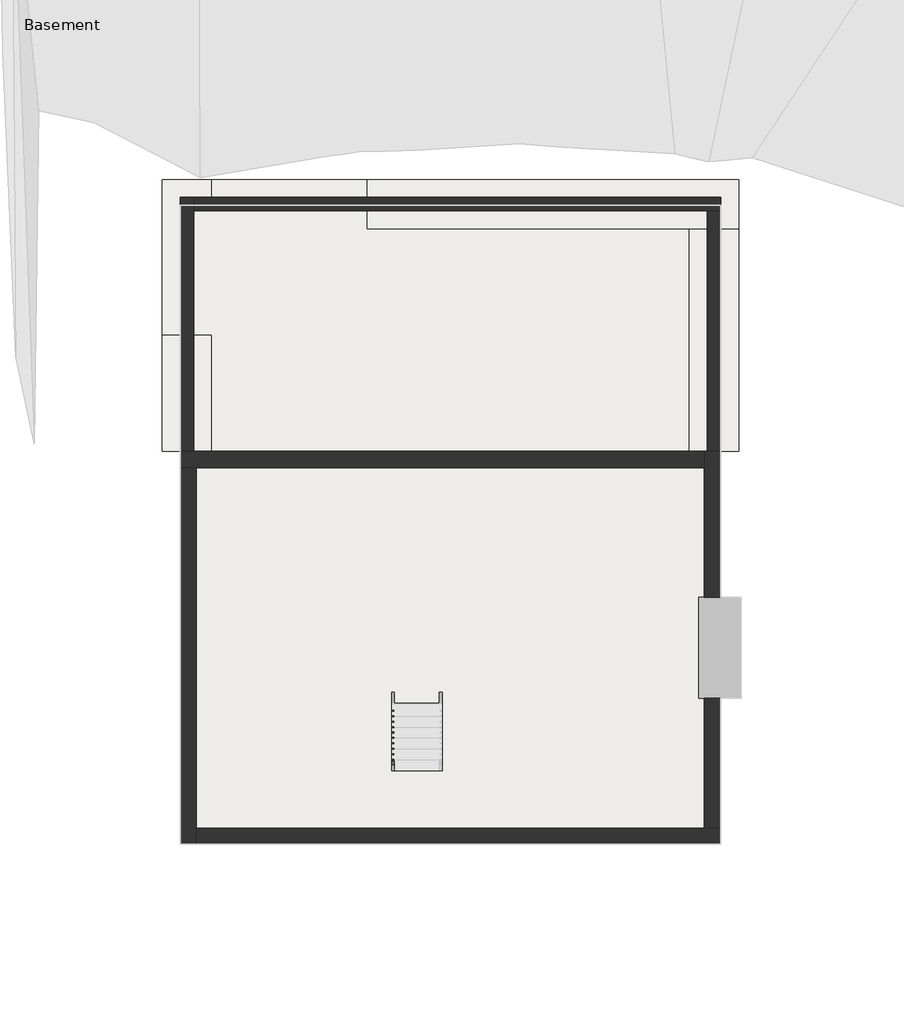
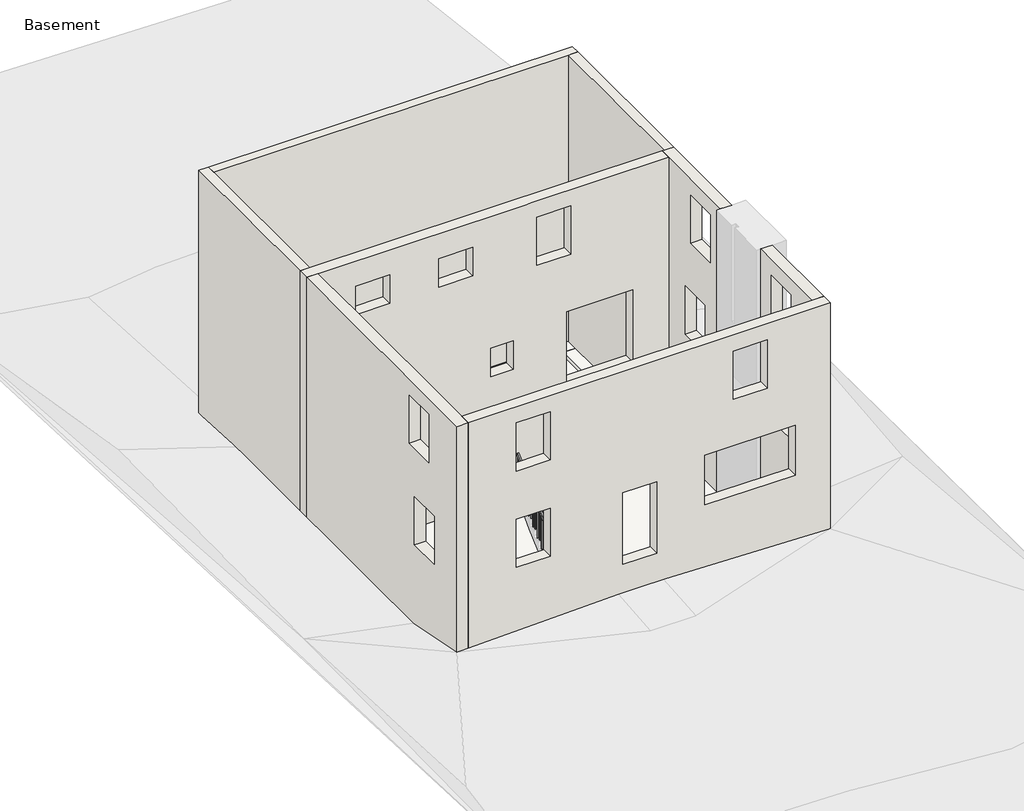
# One storey, part 1 of 2: 8 walls, 3 footings, 2 slabs, 1 railing.
"""IFC4 building model written with IfcOpenShell, lengths in millimetres."""

from ifc_helpers import new_model, si_unit, frame, origin, place, context, project, spatial, polyline, outline, extrude, faceted_brep, element, save

model = new_model("IFC4")

# Units and contexts
model_context = context("Model", 3, world=origin())
ifc_project = project(units=[si_unit("LENGTHUNIT", "METRE", prefix="MILLI")], contexts=[model_context])

# Site, building, storey
site = spatial("IfcSite", under=ifc_project)
building = spatial("IfcBuilding", under=site)
storey = spatial("IfcBuildingStorey", under=building, Name="Basement", Elevation=-2667.0)

# Footings
placement = place(None, origin())
element("IfcFooting", 1, ObjectType="Bearing Footing - 36\" x 12\"", at=placement, inside=storey, context=model_context, shape_type="Brep", body=[
    faceted_brep([(-5404.9803068, 3152.0888758, -2667.0), (-6319.3803068, 3152.0888758, -2667.0), (-6319.3803068, 3152.0888758, -2971.8), (-5404.9803068, 3152.0888758, -2971.8), (-6319.3803068, 5311.0888758, -2667.0), (-5404.9803068, 5311.0888758, -2667.0), (-5404.9803068, 5311.0888758, -2971.8), (-6319.3803068, 5311.0888758, -2971.8)], [[[0, 1, 2, 3]], [[4, 5, 6, 7]], [[0, 5, 4, 1]], [[2, 1, 4, 7]], [[3, 2, 7, 6]], [[0, 3, 6, 5]]]),
    faceted_brep([(-5404.9803068, 5311.0888758, -3124.2), (-6319.3803068, 5311.0888758, -3124.2), (-6319.3803068, 5311.0888758, -3429.0), (-5404.9803068, 5311.0888758, -3429.0), (-5404.9803068, 7292.2888758, -3124.2), (-5404.9803068, 8206.6888758, -3124.2), (-6319.3803068, 8206.6888758, -3124.2), (-6319.3803068, 8206.6888758, -3429.0), (-5404.9803068, 8206.6888758, -3429.0), (-5404.9803068, 7292.2888758, -3429.0)], [[[0, 1, 2, 3]], [[0, 4, 5, 6, 1]], [[2, 1, 6, 7]], [[3, 2, 7, 8, 9]], [[0, 3, 9, 8, 5, 4]], [[6, 5, 8, 7]]]),
])
element("IfcFooting", 2, ObjectType="Bearing Footing - 36\" x 12\"", at=placement, inside=storey, context=model_context, shape_type="Brep", body=[
    faceted_brep([(-2509.3803068, 8206.6888758, -3429.0), (-2509.3803068, 8206.6888758, -3124.2), (-2509.3803068, 7292.2888758, -3124.2), (-2509.3803068, 7292.2888758, -3429.0), (-5404.9803068, 8206.6888758, -3124.2), (-5404.9803068, 7292.2888758, -3124.2), (-5404.9803068, 8206.6888758, -3429.0), (-5404.9803068, 7292.2888758, -3429.0)], [[[0, 1, 2, 3]], [[2, 1, 4, 5]], [[1, 0, 6, 4]], [[0, 3, 7, 6]], [[3, 2, 5, 7]], [[5, 4, 6, 7]]]),
    faceted_brep([(-2509.3803068, 8206.6888758, -2667.0), (-2509.3803068, 8206.6888758, -2971.8), (-2509.3803068, 7292.2888758, -2971.8), (-2509.3803068, 7292.2888758, -2667.0), (4399.4196932, 8206.6888758, -2667.0), (3485.0196932, 7292.2888758, -2667.0), (4399.4196932, 7292.2888758, -2667.0), (4399.4196932, 8206.6888758, -2971.8), (4399.4196932, 7292.2888758, -2971.8), (3485.0196932, 7292.2888758, -2971.8)], [[[0, 1, 2, 3]], [[4, 0, 3, 5, 6]], [[1, 0, 4, 7]], [[2, 1, 7, 8, 9]], [[3, 2, 9, 8, 6, 5]], [[4, 6, 8, 7]]]),
])
element("IfcFooting", 3, ObjectType="Bearing Footing - 36\" x 12\"", at=placement, inside=storey, context=model_context, shape_type="SweptSolid", body=[
    extrude(outline(polyline([(4399.4196932, 3152.0888758), (3485.0196932, 3152.0888758), (3485.0196932, 7292.2888758), (4399.4196932, 7292.2888758), (4399.4196932, 3152.0888758)])), frame((0.0, 0.0, -2971.8), z_axis=(0.0, 0.0, 1.0), x_axis=(1.0, 0.0, 0.0)), (0.0, 0.0, 1.0), 304.8),
])

# Railing
element("IfcRailing", 4, ObjectType="Handrail - Rectangular", at=placement, inside=storey, context=model_context, shape_type="SweptSolid", body=[
    extrude(outline(polyline([(-2791.5111242, -1631.7331862), (-2791.5111242, -1562.1), (-149.9111242, 914.4), (-149.9111242, 844.7668138), (-2791.5111242, -1631.7331862)])), frame((-2052.1803068, 0.0, 0.0), z_axis=(1.0, 0.0, 0.0), x_axis=(0.0, 1.0, 0.0)), (0.0, 0.0, 1.0), 50.8),
    extrude(outline(polyline([(-241.9861242, 758.4465013), (-241.9861242, -190.5), (-261.0361242, -190.5), (-261.0361242, 740.5871263), (-241.9861242, 758.4465013)])), frame((-2036.3053068, 0.0, 0.0), z_axis=(1.0, 0.0, 0.0), x_axis=(0.0, 1.0, 0.0)), (0.0, 0.0, 1.0), 19.05),
    extrude(outline(polyline([(-343.5861242, 663.1965013), (-343.5861242, -190.5), (-362.6361242, -190.5), (-362.6361242, 645.3371263), (-343.5861242, 663.1965013)])), frame((-2036.3053068, 0.0, 0.0), z_axis=(1.0, 0.0, 0.0), x_axis=(0.0, 1.0, 0.0)), (0.0, 0.0, 1.0), 19.05),
    extrude(outline(polyline([(-445.1861242, 567.9465013), (-445.1861242, -381.0), (-464.2361242, -381.0), (-464.2361242, 550.0871263), (-445.1861242, 567.9465013)])), frame((-2036.3053068, 0.0, 0.0), z_axis=(1.0, 0.0, 0.0), x_axis=(0.0, 1.0, 0.0)), (0.0, 0.0, 1.0), 19.05),
    extrude(outline(polyline([(-546.7861242, 472.6965013), (-546.7861242, -381.0), (-565.8361242, -381.0), (-565.8361242, 454.8371263), (-546.7861242, 472.6965013)])), frame((-2036.3053068, 0.0, 0.0), z_axis=(1.0, 0.0, 0.0), x_axis=(0.0, 1.0, 0.0)), (0.0, 0.0, 1.0), 19.05),
    extrude(outline(polyline([(-648.3861242, 377.4465013), (-648.3861242, -571.5), (-667.4361242, -571.5), (-667.4361242, 359.5871263), (-648.3861242, 377.4465013)])), frame((-2036.3053068, 0.0, 0.0), z_axis=(1.0, 0.0, 0.0), x_axis=(0.0, 1.0, 0.0)), (0.0, 0.0, 1.0), 19.05),
    extrude(outline(polyline([(-749.9861242, 282.1965013), (-749.9861242, -571.5), (-769.0361242, -571.5), (-769.0361242, 264.3371263), (-749.9861242, 282.1965013)])), frame((-2036.3053068, 0.0, 0.0), z_axis=(1.0, 0.0, 0.0), x_axis=(0.0, 1.0, 0.0)), (0.0, 0.0, 1.0), 19.05),
    extrude(outline(polyline([(-851.5861242, 186.9465013), (-851.5861242, -762.0), (-870.6361242, -762.0), (-870.6361242, 169.0871263), (-851.5861242, 186.9465013)])), frame((-2036.3053068, 0.0, 0.0), z_axis=(1.0, 0.0, 0.0), x_axis=(0.0, 1.0, 0.0)), (0.0, 0.0, 1.0), 19.05),
    extrude(outline(polyline([(-953.1861242, 91.6965013), (-953.1861242, -762.0), (-972.2361242, -762.0), (-972.2361242, 73.8371263), (-953.1861242, 91.6965013)])), frame((-2036.3053068, 0.0, 0.0), z_axis=(1.0, 0.0, 0.0), x_axis=(0.0, 1.0, 0.0)), (0.0, 0.0, 1.0), 19.05),
    extrude(outline(polyline([(-1054.7861242, -3.5534987), (-1054.7861242, -952.5), (-1073.8361242, -952.5), (-1073.8361242, -21.4128737), (-1054.7861242, -3.5534987)])), frame((-2036.3053068, 0.0, 0.0), z_axis=(1.0, 0.0, 0.0), x_axis=(0.0, 1.0, 0.0)), (0.0, 0.0, 1.0), 19.05),
    extrude(outline(polyline([(-1156.3861242, -98.8034987), (-1156.3861242, -952.5), (-1175.4361242, -952.5), (-1175.4361242, -116.6628737), (-1156.3861242, -98.8034987)])), frame((-2036.3053068, 0.0, 0.0), z_axis=(1.0, 0.0, 0.0), x_axis=(0.0, 1.0, 0.0)), (0.0, 0.0, 1.0), 19.05),
    extrude(outline(polyline([(-1257.9861242, -194.0534987), (-1257.9861242, -1143.0), (-1277.0361242, -1143.0), (-1277.0361242, -211.9128737), (-1257.9861242, -194.0534987)])), frame((-2036.3053068, 0.0, 0.0), z_axis=(1.0, 0.0, 0.0), x_axis=(0.0, 1.0, 0.0)), (0.0, 0.0, 1.0), 19.05),
    extrude(outline(polyline([(-1359.5861242, -289.3034987), (-1359.5861242, -1143.0), (-1378.6361242, -1143.0), (-1378.6361242, -307.1628737), (-1359.5861242, -289.3034987)])), frame((-2036.3053068, 0.0, 0.0), z_axis=(1.0, 0.0, 0.0), x_axis=(0.0, 1.0, 0.0)), (0.0, 0.0, 1.0), 19.05),
    extrude(outline(polyline([(-1461.1861242, -384.5534987), (-1461.1861242, -1333.5), (-1480.2361242, -1333.5), (-1480.2361242, -402.4128737), (-1461.1861242, -384.5534987)])), frame((-2036.3053068, 0.0, 0.0), z_axis=(1.0, 0.0, 0.0), x_axis=(0.0, 1.0, 0.0)), (0.0, 0.0, 1.0), 19.05),
    extrude(outline(polyline([(-1562.7861242, -479.8034987), (-1562.7861242, -1333.5), (-1581.8361242, -1333.5), (-1581.8361242, -497.6628737), (-1562.7861242, -479.8034987)])), frame((-2036.3053068, 0.0, 0.0), z_axis=(1.0, 0.0, 0.0), x_axis=(0.0, 1.0, 0.0)), (0.0, 0.0, 1.0), 19.05),
    extrude(outline(polyline([(-1664.3861242, -575.0534987), (-1664.3861242, -1524.0), (-1683.4361242, -1524.0), (-1683.4361242, -592.9128737), (-1664.3861242, -575.0534987)])), frame((-2036.3053068, 0.0, 0.0), z_axis=(1.0, 0.0, 0.0), x_axis=(0.0, 1.0, 0.0)), (0.0, 0.0, 1.0), 19.05),
    extrude(outline(polyline([(-1765.9861242, -670.3034987), (-1765.9861242, -1524.0), (-1785.0361242, -1524.0), (-1785.0361242, -688.1628737), (-1765.9861242, -670.3034987)])), frame((-2036.3053068, 0.0, 0.0), z_axis=(1.0, 0.0, 0.0), x_axis=(0.0, 1.0, 0.0)), (0.0, 0.0, 1.0), 19.05),
    extrude(outline(polyline([(-1867.5861242, -765.5534987), (-1867.5861242, -1714.5), (-1886.6361242, -1714.5), (-1886.6361242, -783.4128737), (-1867.5861242, -765.5534987)])), frame((-2036.3053068, 0.0, 0.0), z_axis=(1.0, 0.0, 0.0), x_axis=(0.0, 1.0, 0.0)), (0.0, 0.0, 1.0), 19.05),
    extrude(outline(polyline([(-1969.1861242, -860.8034987), (-1969.1861242, -1714.5), (-1988.2361242, -1714.5), (-1988.2361242, -878.6628737), (-1969.1861242, -860.8034987)])), frame((-2036.3053068, 0.0, 0.0), z_axis=(1.0, 0.0, 0.0), x_axis=(0.0, 1.0, 0.0)), (0.0, 0.0, 1.0), 19.05),
    extrude(outline(polyline([(-2070.7861242, -956.0534987), (-2070.7861242, -1905.0), (-2089.8361242, -1905.0), (-2089.8361242, -973.9128737), (-2070.7861242, -956.0534987)])), frame((-2036.3053068, 0.0, 0.0), z_axis=(1.0, 0.0, 0.0), x_axis=(0.0, 1.0, 0.0)), (0.0, 0.0, 1.0), 19.05),
    extrude(outline(polyline([(-2172.3861242, -1051.3034987), (-2172.3861242, -1905.0), (-2191.4361242, -1905.0), (-2191.4361242, -1069.1628737), (-2172.3861242, -1051.3034987)])), frame((-2036.3053068, 0.0, 0.0), z_axis=(1.0, 0.0, 0.0), x_axis=(0.0, 1.0, 0.0)), (0.0, 0.0, 1.0), 19.05),
    extrude(outline(polyline([(-2273.9861242, -1146.5534987), (-2273.9861242, -2095.5), (-2293.0361242, -2095.5), (-2293.0361242, -1164.4128737), (-2273.9861242, -1146.5534987)])), frame((-2036.3053068, 0.0, 0.0), z_axis=(1.0, 0.0, 0.0), x_axis=(0.0, 1.0, 0.0)), (0.0, 0.0, 1.0), 19.05),
    extrude(outline(polyline([(-2375.5861242, -1241.8034987), (-2375.5861242, -2095.5), (-2394.6361242, -2095.5), (-2394.6361242, -1259.6628737), (-2375.5861242, -1241.8034987)])), frame((-2036.3053068, 0.0, 0.0), z_axis=(1.0, 0.0, 0.0), x_axis=(0.0, 1.0, 0.0)), (0.0, 0.0, 1.0), 19.05),
    extrude(outline(polyline([(-2477.1861242, -1337.0534987), (-2477.1861242, -2286.0), (-2496.2361242, -2286.0), (-2496.2361242, -1354.9128737), (-2477.1861242, -1337.0534987)])), frame((-2036.3053068, 0.0, 0.0), z_axis=(1.0, 0.0, 0.0), x_axis=(0.0, 1.0, 0.0)), (0.0, 0.0, 1.0), 19.05),
    extrude(outline(polyline([(-2578.7861242, -1432.3034987), (-2578.7861242, -2286.0), (-2597.8361242, -2286.0), (-2597.8361242, -1450.1628737), (-2578.7861242, -1432.3034987)])), frame((-2036.3053068, 0.0, 0.0), z_axis=(1.0, 0.0, 0.0), x_axis=(0.0, 1.0, 0.0)), (0.0, 0.0, 1.0), 19.05),
    extrude(outline(polyline([(-2680.3861242, -1527.5534987), (-2680.3861242, -2476.5), (-2699.4361242, -2476.5), (-2699.4361242, -1545.4128737), (-2680.3861242, -1527.5534987)])), frame((-2036.3053068, 0.0, 0.0), z_axis=(1.0, 0.0, 0.0), x_axis=(0.0, 1.0, 0.0)), (0.0, 0.0, 1.0), 19.05),
    extrude(outline(polyline([(-149.9111242, 844.7668138), (-149.9111242, -190.5), (-168.9611242, -190.5), (-168.9611242, 826.9074388), (-149.9111242, 844.7668138)])), frame((-2036.3053068, 0.0, 0.0), z_axis=(1.0, 0.0, 0.0), x_axis=(0.0, 1.0, 0.0)), (0.0, 0.0, 1.0), 19.05),
    extrude(outline(polyline([(-2772.4611242, -1613.8738112), (-2772.4611242, -2476.5), (-2791.5111242, -2476.5), (-2791.5111242, -1631.7331862), (-2772.4611242, -1613.8738112)])), frame((-2036.3053068, 0.0, 0.0), z_axis=(1.0, 0.0, 0.0), x_axis=(0.0, 1.0, 0.0)), (0.0, 0.0, 1.0), 19.05),
])

# Slabs
element("IfcSlab", 5, ObjectType="Pad 1", at=placement, inside=storey, context=model_context, shape_type="SweptSolid", body=[
    extrude(outline(polyline([(4069.2196932, 434.2888758), (4450.2196932, 434.2888758), (4450.2196932, -1445.3111242), (4069.2196932, -1445.3111242), (4069.2196932, -4163.1111242), (-5989.1803068, -4163.1111242), (-5989.1803068, 3152.0888758), (4069.2196932, 3152.0888758), (4069.2196932, 434.2888758)])), frame((0.0, 0.0, -3073.4), z_axis=(0.0, 0.0, 1.0), x_axis=(1.0, 0.0, 0.0)), (0.0, 0.0, 1.0), 304.8),
])
element("IfcSlab", 6, ObjectType="Pad 1", at=placement, inside=storey, context=model_context, shape_type="SweptSolid", body=[
    extrude(outline(polyline([(-5989.1803068, 7724.0888758), (4069.2196932, 7724.0888758), (4069.2196932, 3152.0888758), (-5989.1803068, 3152.0888758), (-5989.1803068, 7724.0888758)])), frame((0.0, 0.0, -3073.4), z_axis=(0.0, 0.0, 1.0), x_axis=(1.0, 0.0, 0.0)), (0.0, 0.0, 1.0), 304.8),
])

# Walls
element("IfcWall", 7, ObjectType="Generic - 10\"", at=placement, inside=storey, context=model_context, shape_type="Brep", body=[
    faceted_brep([(-5735.1803068, 3152.0888758, -2667.0), (-5735.1803068, 5311.0888758, -2667.0), (-5735.1803068, 5311.0888758, -3124.2), (-5735.1803068, 7622.4888758, -3124.2), (-5735.1803068, 7876.4888758, -3124.2), (-5735.1803068, 7876.4888758, 5486.4), (-5735.1803068, 7622.4888758, 5486.4), (-5735.1803068, 3152.0888758, 5486.4), (-5989.1803068, 3152.0888758, -2667.0), (-5989.1803068, 3152.0888758, 5486.4), (-5989.1803068, 7876.4888758, 5486.4), (-5989.1803068, 7876.4888758, -3124.2), (-5989.1803068, 5311.0888758, -3124.2), (-5989.1803068, 5311.0888758, -2667.0)], [[[0, 1, 2, 3, 4, 5, 6, 7]], [[8, 9, 10, 11, 12, 13]], [[1, 0, 8, 13]], [[2, 1, 13, 12]], [[4, 3, 2, 12, 11]], [[7, 6, 5, 10, 9]], [[5, 4, 11, 10]], [[0, 7, 9, 8]]]),
])
element("IfcWall", 8, ObjectType="Generic - 10\"", at=placement, inside=storey, context=model_context, shape_type="Brep", body=[
    faceted_brep([(-5735.1803068, 7622.4888758, -3124.2), (-2509.3803068, 7622.4888758, -3124.2), (-2509.3803068, 7622.4888758, -2667.0), (3815.2196932, 7622.4888758, -2667.0), (4069.2196932, 7622.4888758, -2667.0), (4069.2196932, 7622.4888758, 5486.4), (3815.2196932, 7622.4888758, 5486.4), (-5735.1803068, 7622.4888758, 5486.4), (-5735.1803068, 7876.4888758, -3124.2), (-5735.1803068, 7876.4888758, 5486.4), (4069.2196932, 7876.4888758, 5486.4), (4069.2196932, 7876.4888758, -2667.0), (-2509.3803068, 7876.4888758, -2667.0), (-2509.3803068, 7876.4888758, -3124.2)], [[[0, 1, 2, 3, 4, 5, 6, 7]], [[8, 9, 10, 11, 12, 13]], [[1, 0, 8, 13]], [[2, 1, 13, 12]], [[4, 3, 2, 12, 11]], [[7, 6, 5, 10, 9]], [[5, 4, 11, 10]], [[0, 7, 9, 8]]]),
])
element("IfcWall", 9, ObjectType="Generic - 10\"", at=placement, inside=storey, context=model_context, shape_type="SweptSolid", body=[
    extrude(outline(polyline([(3815.2196932, 3152.0888758), (3815.2196932, 7622.4888758), (4069.2196932, 7622.4888758), (4069.2196932, 3152.0888758), (3815.2196932, 3152.0888758)])), frame((0.0, 0.0, -2667.0), z_axis=(0.0, 0.0, 1.0), x_axis=(1.0, 0.0, 0.0)), (0.0, 0.0, 1.0), 8153.4),
])
element("IfcWall", 10, ObjectType="Generic - 12\"", at=placement, inside=storey, context=model_context, shape_type="Brep", body=[
    faceted_brep([(-5989.1803068, 2847.2888758, -2667.0), (-5684.3803068, 2847.2888758, -2667.0), (3764.4196932, 2847.2888758, -2667.0), (3764.4196932, 2847.2888758, 5486.4), (56.0196932, 2847.2888758, 5486.4), (-70.9803068, 2847.2888758, 5486.4), (-680.5803068, 2847.2888758, 5486.4), (-807.5803068, 2847.2888758, 5486.4), (-3169.7803068, 2847.2888758, 5486.4), (-3296.7803068, 2847.2888758, 5486.4), (-5684.3803068, 2847.2888758, 5486.4), (-5989.1803068, 2847.2888758, 5486.4), (1021.2196932, 2847.2888758, 0.0), (1021.2196932, 2847.2888758, 2057.4), (2799.2196932, 2847.2888758, 2057.4), (2799.2196932, 2847.2888758, 0.0), (-4160.3803068, 2847.2888758, 0.0), (-5023.9803068, 2847.2888758, 0.0), (-5023.9803068, 2847.2888758, 2032.0), (-4160.3803068, 2847.2888758, 2032.0), (-1036.1803068, 2847.2888758, 914.4), (-1036.1803068, 2847.2888758, 1727.2), (-426.5803068, 2847.2888758, 1727.2), (-426.5803068, 2847.2888758, 914.4), (-3919.0803068, 2847.2888758, 914.4), (-3919.0803068, 2847.2888758, 1727.2), (-3004.6803068, 2847.2888758, 1727.2), (-3004.6803068, 2847.2888758, 914.4), (208.4196932, 2847.2888758, 3657.6), (208.4196932, 2847.2888758, 5029.2), (1122.8196932, 2847.2888758, 5029.2), (1122.8196932, 2847.2888758, 3657.6), (-2433.1803068, 2847.2888758, 3962.4), (-2433.1803068, 2847.2888758, 4775.2), (-1518.7803068, 2847.2888758, 4775.2), (-1518.7803068, 2847.2888758, 3962.4), (-4668.3803068, 2847.2888758, 3962.4), (-4668.3803068, 2847.2888758, 4775.2), (-3753.9803068, 2847.2888758, 4775.2), (-3753.9803068, 2847.2888758, 3962.4), (3764.4196932, 3152.0888758, -2667.0), (-5989.1803068, 3152.0888758, -2667.0), (-5989.1803068, 3152.0888758, 5486.4), (3764.4196932, 3152.0888758, 5486.4), (1021.2196932, 3152.0888758, 2057.4), (1021.2196932, 3152.0888758, 0.0), (2799.2196932, 3152.0888758, 0.0), (2799.2196932, 3152.0888758, 2057.4), (-5023.9803068, 3152.0888758, 0.0), (-4160.3803068, 3152.0888758, 0.0), (-4160.3803068, 3152.0888758, 2032.0), (-5023.9803068, 3152.0888758, 2032.0), (-1036.1803068, 3152.0888758, 1727.2), (-1036.1803068, 3152.0888758, 914.4), (-426.5803068, 3152.0888758, 914.4), (-426.5803068, 3152.0888758, 1727.2), (-3919.0803068, 3152.0888758, 1727.2), (-3919.0803068, 3152.0888758, 914.4), (-3004.6803068, 3152.0888758, 914.4), (-3004.6803068, 3152.0888758, 1727.2), (208.4196932, 3152.0888758, 5029.2), (208.4196932, 3152.0888758, 3657.6), (1122.8196932, 3152.0888758, 3657.6), (1122.8196932, 3152.0888758, 5029.2), (-2433.1803068, 3152.0888758, 4775.2), (-2433.1803068, 3152.0888758, 3962.4), (-1518.7803068, 3152.0888758, 3962.4), (-1518.7803068, 3152.0888758, 4775.2), (-4668.3803068, 3152.0888758, 4775.2), (-4668.3803068, 3152.0888758, 3962.4), (-3753.9803068, 3152.0888758, 3962.4), (-3753.9803068, 3152.0888758, 4775.2)], [[[0, 1, 2, 3, 4, 5, 6, 7, 8, 9, 10, 11], [12, 13, 14, 15], [16, 17, 18, 19], [20, 21, 22, 23], [24, 25, 26, 27], [28, 29, 30, 31], [32, 33, 34, 35], [36, 37, 38, 39]], [[40, 41, 42, 43], [44, 45, 46, 47], [48, 49, 50, 51], [52, 53, 54, 55], [56, 57, 58, 59], [60, 61, 62, 63], [64, 65, 66, 67], [68, 69, 70, 71]], [[2, 1, 0, 41, 40]], [[11, 10, 9, 8, 7, 6, 5, 4, 3, 43, 42]], [[0, 11, 42, 41]], [[3, 2, 40, 43]], [[44, 13, 12, 45]], [[13, 44, 47, 14]], [[14, 47, 46, 15]], [[45, 12, 15, 46]], [[17, 16, 49, 48]], [[18, 17, 48, 51]], [[19, 18, 51, 50]], [[16, 19, 50, 49]], [[53, 52, 21, 20]], [[54, 53, 20, 23]], [[55, 54, 23, 22]], [[52, 55, 22, 21]], [[57, 56, 25, 24]], [[58, 57, 24, 27]], [[59, 58, 27, 26]], [[56, 59, 26, 25]], [[60, 29, 28, 61]], [[61, 28, 31, 62]], [[62, 31, 30, 63]], [[29, 60, 63, 30]], [[33, 32, 65, 64]], [[32, 35, 66, 65]], [[35, 34, 67, 66]], [[34, 33, 64, 67]], [[37, 36, 69, 68]], [[36, 39, 70, 69]], [[39, 38, 71, 70]], [[38, 37, 68, 71]]]),
])
element("IfcWall", 11, ObjectType="Generic - 12\"", at=placement, inside=storey, context=model_context, shape_type="Brep", body=[
    faceted_brep([(-5684.3803068, -4163.1111242, -2667.0), (-5684.3803068, -3858.3111242, -2667.0), (-5684.3803068, 2847.2888758, -2667.0), (-5684.3803068, 2847.2888758, 5486.4), (-5684.3803068, 1450.2888758, 5486.4), (-5684.3803068, 1323.2888758, 5486.4), (-5684.3803068, -3858.3111242, 5486.4), (-5684.3803068, -4163.1111242, 5486.4), (-5684.3803068, -3096.3111242, 914.4), (-5684.3803068, -3096.3111242, 2286.0), (-5684.3803068, -2181.9111242, 2286.0), (-5684.3803068, -2181.9111242, 914.4), (-5684.3803068, -2842.3111242, 3657.6), (-5684.3803068, -2842.3111242, 5029.2), (-5684.3803068, -1927.9111242, 5029.2), (-5684.3803068, -1927.9111242, 3657.6), (-5989.1803068, 2847.2888758, -2667.0), (-5989.1803068, -4163.1111242, -2667.0), (-5989.1803068, -4163.1111242, 5486.4), (-5989.1803068, 2847.2888758, 5486.4), (-5989.1803068, -3096.3111242, 2286.0), (-5989.1803068, -3096.3111242, 914.4), (-5989.1803068, -2181.9111242, 914.4), (-5989.1803068, -2181.9111242, 2286.0), (-5989.1803068, -2842.3111242, 5029.2), (-5989.1803068, -2842.3111242, 3657.6), (-5989.1803068, -1927.9111242, 3657.6), (-5989.1803068, -1927.9111242, 5029.2)], [[[0, 1, 2, 3, 4, 5, 6, 7], [8, 9, 10, 11], [12, 13, 14, 15]], [[16, 17, 18, 19], [20, 21, 22, 23], [24, 25, 26, 27]], [[2, 1, 0, 17, 16]], [[7, 6, 5, 4, 3, 19, 18]], [[0, 7, 18, 17]], [[3, 2, 16, 19]], [[21, 20, 9, 8]], [[22, 21, 8, 11]], [[23, 22, 11, 10]], [[20, 23, 10, 9]], [[24, 13, 12, 25]], [[25, 12, 15, 26]], [[26, 15, 14, 27]], [[13, 24, 27, 14]]]),
])
element("IfcWall", 12, ObjectType="Generic - 12\"", at=placement, inside=storey, context=model_context, shape_type="Brep", body=[
    faceted_brep([(4069.2196932, -3858.3111242, -2667.0), (3764.4196932, -3858.3111242, -2667.0), (-5684.3803068, -3858.3111242, -2667.0), (-5684.3803068, -3858.3111242, 5486.4), (-2179.1803068, -3858.3111242, 5486.4), (-2052.1803068, -3858.3111242, 5486.4), (-807.5803068, -3858.3111242, 5486.4), (-680.5803068, -3858.3111242, 5486.4), (-70.9803068, -3858.3111242, 5486.4), (56.0196932, -3858.3111242, 5486.4), (3764.4196932, -3858.3111242, 5486.4), (4069.2196932, -3858.3111242, 5486.4), (-1518.7803068, -3858.3111242, 0.0), (-604.3803068, -3858.3111242, 0.0), (-604.3803068, -3858.3111242, 2032.0), (-1518.7803068, -3858.3111242, 2032.0), (-3474.5803068, -3858.3111242, 914.4), (-3474.5803068, -3858.3111242, 2286.0), (-4388.9803068, -3858.3111242, 2286.0), (-4388.9803068, -3858.3111242, 914.4), (2367.4196932, -3858.3111242, 3657.6), (2367.4196932, -3858.3111242, 5029.2), (1453.0196932, -3858.3111242, 5029.2), (1453.0196932, -3858.3111242, 3657.6), (-3474.5803068, -3858.3111242, 3657.6), (-3474.5803068, -3858.3111242, 5029.2), (-4388.9803068, -3858.3111242, 5029.2), (-4388.9803068, -3858.3111242, 3657.6), (3129.4196932, -3858.3111242, 2336.8), (691.0196932, -3858.3111242, 2336.8), (691.0196932, -3858.3111242, 914.4), (3129.4196932, -3858.3111242, 914.4), (-5684.3803068, -4163.1111242, -2667.0), (4069.2196932, -4163.1111242, -2667.0), (4069.2196932, -4163.1111242, 5486.4), (-5684.3803068, -4163.1111242, 5486.4), (-604.3803068, -4163.1111242, 0.0), (-1518.7803068, -4163.1111242, 0.0), (-1518.7803068, -4163.1111242, 2032.0), (-604.3803068, -4163.1111242, 2032.0), (-3474.5803068, -4163.1111242, 2286.0), (-3474.5803068, -4163.1111242, 914.4), (-4388.9803068, -4163.1111242, 914.4), (-4388.9803068, -4163.1111242, 2286.0), (2367.4196932, -4163.1111242, 5029.2), (2367.4196932, -4163.1111242, 3657.6), (1453.0196932, -4163.1111242, 3657.6), (1453.0196932, -4163.1111242, 5029.2), (-3474.5803068, -4163.1111242, 5029.2), (-3474.5803068, -4163.1111242, 3657.6), (-4388.9803068, -4163.1111242, 3657.6), (-4388.9803068, -4163.1111242, 5029.2), (3129.4196932, -4163.1111242, 914.4), (691.0196932, -4163.1111242, 914.4), (691.0196932, -4163.1111242, 2336.8), (3129.4196932, -4163.1111242, 2336.8)], [[[0, 1, 2, 3, 4, 5, 6, 7, 8, 9, 10, 11], [12, 13, 14, 15], [16, 17, 18, 19], [20, 21, 22, 23], [24, 25, 26, 27], [28, 29, 30, 31]], [[32, 33, 34, 35], [36, 37, 38, 39], [40, 41, 42, 43], [44, 45, 46, 47], [48, 49, 50, 51], [52, 53, 54, 55]], [[2, 1, 0, 33, 32]], [[11, 10, 9, 8, 7, 6, 5, 4, 3, 35, 34]], [[0, 11, 34, 33]], [[3, 2, 32, 35]], [[37, 36, 13, 12]], [[38, 37, 12, 15]], [[39, 38, 15, 14]], [[36, 39, 14, 13]], [[41, 40, 17, 16]], [[42, 41, 16, 19]], [[43, 42, 19, 18]], [[40, 43, 18, 17]], [[30, 53, 52, 31]], [[54, 29, 28, 55]], [[29, 54, 53, 30]], [[31, 52, 55, 28]], [[21, 20, 45, 44]], [[20, 23, 46, 45]], [[23, 22, 47, 46]], [[22, 21, 44, 47]], [[25, 24, 49, 48]], [[24, 27, 50, 49]], [[27, 26, 51, 50]], [[26, 25, 48, 51]]]),
])
element("IfcWall", 13, ObjectType="Generic - 12\"", at=placement, inside=storey, context=model_context, shape_type="Brep", body=[
    faceted_brep([(3764.4196932, 3152.0888758, -2667.0), (3764.4196932, 2847.2888758, -2667.0), (3764.4196932, 434.2888758, -2667.0), (3764.4196932, 434.2888758, 5486.4), (3764.4196932, 2847.2888758, 5486.4), (3764.4196932, 3152.0888758, 5486.4), (3764.4196932, 2085.2888758, 914.4), (3764.4196932, 2085.2888758, 2286.0), (3764.4196932, 1170.8888758, 2286.0), (3764.4196932, 1170.8888758, 914.4), (3764.4196932, 1831.2888758, 3657.6), (3764.4196932, 1831.2888758, 5029.2), (3764.4196932, 916.8888758, 5029.2), (3764.4196932, 916.8888758, 3657.6), (4069.2196932, 434.2888758, -2667.0), (4069.2196932, 3152.0888758, -2667.0), (4069.2196932, 3152.0888758, 5486.4), (4069.2196932, 434.2888758, 5486.4), (4069.2196932, 2085.2888758, 2286.0), (4069.2196932, 2085.2888758, 914.4), (4069.2196932, 1170.8888758, 914.4), (4069.2196932, 1170.8888758, 2286.0), (4069.2196932, 1831.2888758, 5029.2), (4069.2196932, 1831.2888758, 3657.6), (4069.2196932, 916.8888758, 3657.6), (4069.2196932, 916.8888758, 5029.2)], [[[0, 1, 2, 3, 4, 5], [6, 7, 8, 9], [10, 11, 12, 13]], [[14, 15, 16, 17], [18, 19, 20, 21], [22, 23, 24, 25]], [[2, 1, 0, 15, 14]], [[3, 2, 14, 17]], [[5, 4, 3, 17, 16]], [[0, 5, 16, 15]], [[19, 18, 7, 6]], [[20, 19, 6, 9]], [[21, 20, 9, 8]], [[18, 21, 8, 7]], [[22, 11, 10, 23]], [[23, 10, 13, 24]], [[24, 13, 12, 25]], [[11, 22, 25, 12]]]),
])
element("IfcWall", 14, ObjectType="Generic - 12\"", at=placement, inside=storey, context=model_context, shape_type="SweptSolid", body=[
    extrude(outline(polyline([(-1445.3111242, -2667.0), (-3858.3111242, -2667.0), (-3858.3111242, 5486.4), (-1445.3111242, 5486.4), (-1445.3111242, -2667.0)]), holes=[polyline([(-2181.9111242, 2286.0), (-3096.3111242, 2286.0), (-3096.3111242, 914.4), (-2181.9111242, 914.4), (-2181.9111242, 2286.0)]), polyline([(-1927.9111242, 3657.6), (-1927.9111242, 5029.2), (-2842.3111242, 5029.2), (-2842.3111242, 3657.6), (-1927.9111242, 3657.6)])]), frame((3764.4196932, 0.0, 0.0), z_axis=(1.0, 0.0, 0.0), x_axis=(0.0, 1.0, 0.0)), (0.0, 0.0, 1.0), 304.8),
])

save(model, "model.ifc")

# Revit data of these elements
# Project information
#   Organization Name = "G3B Press"
#   Organization Description = "Paul F. Aubin Cosulting Services, Inc."
#   Building Name = "Revit Essentials for Architecture"
#   Author = "Paul F. Aubin"
#   Author Website = "https://www.paulaubin.com"
#   Copyright = "Copyright © 2020 Paul F Aubin, all rights reserved"
#   Project Issue Date = "8/1/2020"
#   Project Status = "Design Development"
#   Client Name = "Floors and Roofs"
#   Project Address = "789 Main ST\nAnytown, IL 60000"
#   Project Name = "09 Residential"
#   Project Number = "2020.03A"
# Type "Bearing Footing - 36\" x 12\""
#   Assembly Code = "A1010110"
# Type "Handrail - Rectangular"
#   Assembly Code = "C2010400"
#   built-in parameter 1008612 = 0.0416667 (stored number, unit not read)
#   built-in parameter 1008611 = 0.0416667 (stored number, unit not read)
#   built-in parameter 1008609 = 0.333333 (stored number, unit not read)
#   built-in parameter 1008604 = 0.166667 (stored number, unit not read)
#   built-in parameter 1008603 = 0.166667 (stored number, unit not read)
#   Railing Height = 3' - 0"
#   built-in parameter 1008630 = 2
#   built-in parameter 1008610 = 2
#   built-in parameter 1008618 = Baluster - Square : 3/4"
# Type "Pad 1"
#   Layers, outside or top first: 1' - 0" no material (function 1)
# Type "Generic - 10\""
#   Assembly Code = "B2010"
#   Layers, outside or top first: 0' - 10" no material (function 1)
# Type "Generic - 12\""
#   Assembly Code = "B2010"
#   Layers, outside or top first: 1' - 0" no material (function 1)
# Element 1 (IfcFooting, "Bearing Footing - 36\" x 12\"")
#   Phase Created = New Construction
#   Materials on its faces: "Concrete, Cast-in-Place gray"
# Elements 2, 3 (IfcFooting, "Bearing Footing - 36\" x 12\"")
#   Comments = ""
#   Phase Created = New Construction
#   Materials on its faces: "Concrete, Cast-in-Place gray"
# Element 4 (IfcRailing, "Handrail - Rectangular")
#   Phase Created = Existing
# Elements 5, 6 (IfcSlab, "Pad 1")
#   built-in parameter 1012502 = -0.333333 (stored number, unit not read)
#   Phase Created = New Construction
# Elements 7, 8, 9 (IfcWall, "Generic - 10\"")
#   Top Offset = 0' - 0"
#   Base Offset = 0' - 0"
#   wall height = 26' - 9"
#   Phase Created = New Construction
#   Base Constraint = Basement
#   Top Constraint = Roof
#   Materials on its faces: "Default Wall"
# Elements 10, 11, 12, 13, 14 (IfcWall, "Generic - 12\"")
#   Top Offset = 0' - 0"
#   Base Offset = 0' - 0"
#   wall height = 26' - 9"
#   Phase Created = Existing
#   Base Constraint = Basement
#   Top Constraint = Roof
#   Materials on its faces: "Default Wall"
# Materials
#   "Concrete, Cast-in-Place gray": class "Concrete", colour RGB 192 192 192, transparency 0, Description = "Cast-in-place concrete", Cost = 0
#   "Default Wall": class "Miscellaneous", colour RGB 128 128 128, transparency 0, Cost = 0
